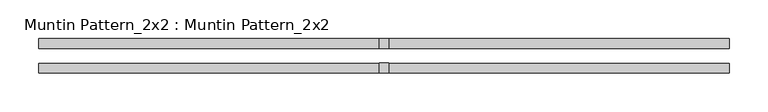
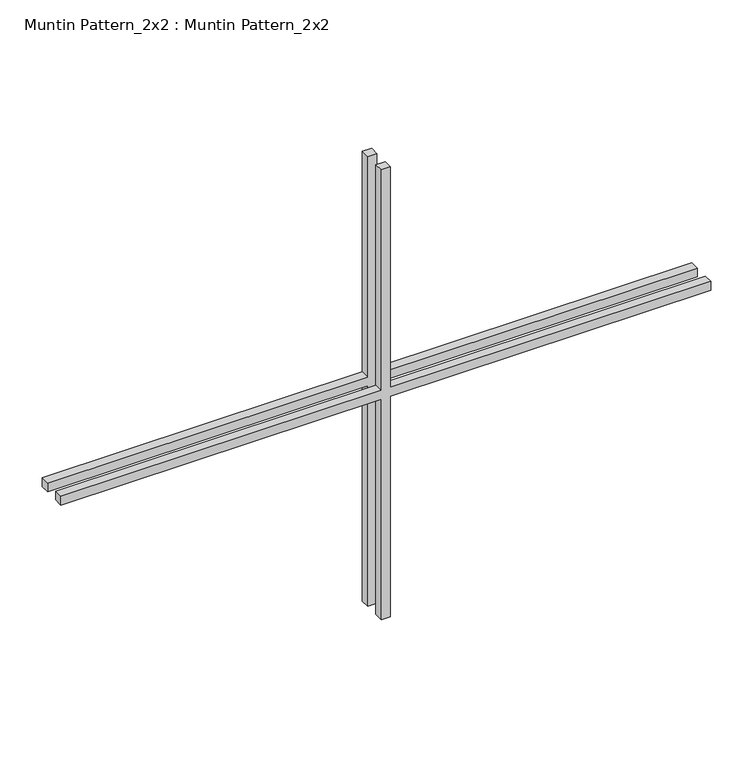
"""IFC4 building model written with IfcOpenShell, lengths in millimetres: proxy geometry, Muntin Pattern_2x2 : Muntin Pattern_2x2."""

from ifc_helpers import new_model, si_unit, frame, origin, place, context, project, spatial, polyline, outline, extrude, source, transform, mapped, element, save


def muntin_pattern_2x2_muntin_pattern_2x2_e308e741(model_context):
    return source(origin(), model_context, "Body", "SweptSolid", [
        extrude(outline(polyline([(331.7875, -6.35), (331.7875, -444.5), (319.0875, -444.5), (319.0875, -6.35), (0.0, -6.35), (0.0, 6.35), (319.0875, 6.35), (319.0875, 444.5), (331.7875, 444.5), (331.7875, 6.35), (650.875, 6.35), (650.875, -6.35), (331.7875, -6.35)])), frame((0.0, -22.225, 0.0), z_axis=(0.0, 1.0, 0.0), x_axis=(0.0, 0.0, 1.0)), (0.0, 0.0, 1.0), 12.7),
        extrude(outline(polyline([(331.7875, -6.35), (331.7875, -444.5), (319.0875, -444.5), (319.0875, -6.35), (0.0, -6.35), (0.0, 6.35), (319.0875, 6.35), (319.0875, 444.5), (331.7875, 444.5), (331.7875, 6.35), (650.875, 6.35), (650.875, -6.35), (331.7875, -6.35)])), frame((0.0, 9.525, 0.0), z_axis=(0.0, 1.0, 0.0), x_axis=(0.0, 0.0, 1.0)), (0.0, 0.0, 1.0), 12.7),
    ])


if __name__ == "__main__":
    model = new_model("IFC4")
    model_context = context("Model", 3, world=origin())
    ifc_project = project(units=[si_unit("LENGTHUNIT", "METRE", prefix="MILLI")], contexts=[model_context])
    site = spatial("IfcSite", under=ifc_project)
    building = spatial("IfcBuilding", under=site)
    placement = place(None, origin())
    muntin_pattern_2x2_muntin_pattern_2x2_shape = muntin_pattern_2x2_muntin_pattern_2x2_e308e741(model_context)
    element("IfcBuildingElementProxy", 1, Name="Muntin Pattern_2x2 : Muntin Pattern_2x2", ObjectType="Muntin Pattern_2x2 : Muntin Pattern_2x2", at=placement, inside=building, context=model_context, shape_type="MappedRepresentation", body=[
        mapped(muntin_pattern_2x2_muntin_pattern_2x2_shape, transform((0.0, 0.0, 0.0), x_axis=(1.0, 0.0, 0.0), y_axis=(0.0, 1.0, 0.0), z_axis=(0.0, 0.0, 1.0))),
    ])
    save(model, "model.ifc")

# Revit data of these elements
# Type "Muntin Pattern_2x2 : Muntin Pattern_2x2"
#   Width [instance default] = 4' - 0"
#   Thickness = 0' - 0 1/2"
#   Height [instance default] = 4' - 0"
#   Distance = 0' - 0 3/4"
#   Interior Material [instance default] = none
#   Exterior Material [instance default] = none
# Element 1 (IfcBuildingElementProxy, "Muntin Pattern_2x2 : Muntin Pattern_2x2")
#   Width = 2' - 11"
#   Height = 2' - 1 5/8"
#   Interior Material = Wood - Stained
#   Exterior Material = Clad - White
#   Materials on its faces: "Clad - White", "Wood - Stained"
# Materials
#   "Clad - White": class "Wood", colour RGB 242 242 238, transparency 0, Cost = 0
#   "Wood - Stained": class "Wood", colour RGB 224 178 126, transparency 0, Cost = 0
